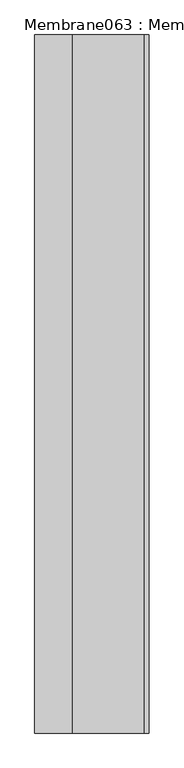
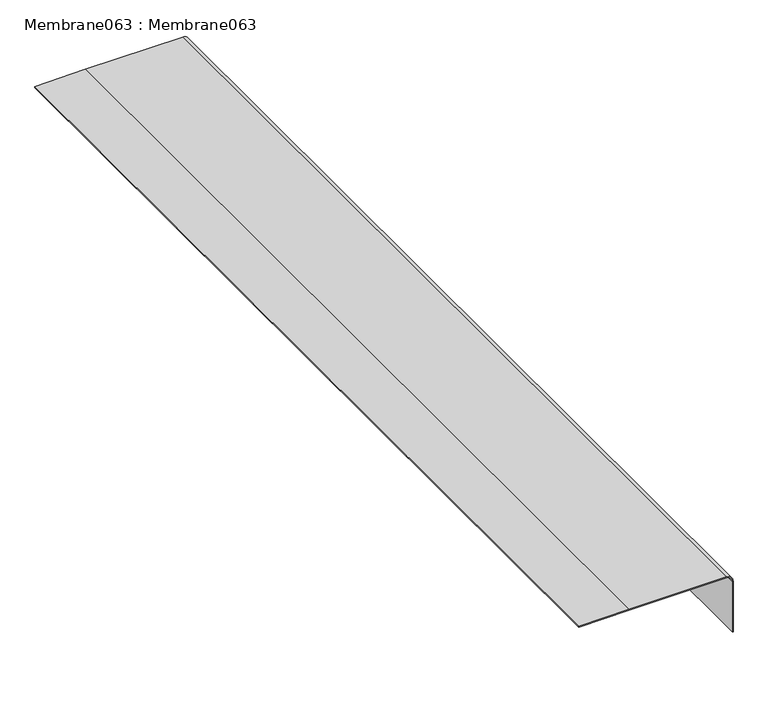
"""IFC4 building model written with IfcOpenShell, lengths in millimetres: proxy geometry, Membrane063 : Membrane063."""

from ifc_helpers import new_model, si_unit, point, frame, frame_2d, origin, place, context, project, spatial, polyline, circle_curve, trimmed, segment, composite_curve, outline, extrude, source, transform, mapped, element, save


def membrane063_membrane063_a49dec39(model_context):
    return source(origin(), model_context, "Body", "SweptSolid", [
        extrude(outline(composite_curve([segment(polyline([(40234.5370749, -4374.0545197), (40120.9129128, -4374.0545197), (40120.9129128, -4372.0545197), (40234.5370749, -4372.0545197)]), True, "CONTINUOUS"), segment(trimmed(circle_curve(frame_2d((40234.5370749, -4386.0545197)), 14.0), [point((40234.5370749, -4372.0545197))], [point((40248.5370749, -4386.0545197))], False, "CARTESIAN"), True, "CONTINUOUS"), segment(polyline([(40248.5370749, -4386.0545197), (40248.5370749, -4593.337414), (40247.0048323, -4699.8063764), (40245.0046252, -4699.8063764), (40246.5370749, -4593.3230233), (40246.5370749, -4386.0545197)]), True, "CONTINUOUS"), segment(trimmed(circle_curve(frame_2d((40234.5370749, -4386.0545197)), 12.0), [point((40246.5370749, -4386.0545197))], [point((40234.5370749, -4374.0545197))], True, "CARTESIAN"), True, "CONTINUOUS")], self_intersect=False)), frame((0.0, -1052.8906574, 0.0), z_axis=(0.0, 1.0, 0.0), x_axis=(0.0, 0.0, 1.0)), (0.0, 0.0, 1.0), 2000.0),
    ])


if __name__ == "__main__":
    model = new_model("IFC4")
    model_context = context("Model", 3, world=origin())
    ifc_project = project(units=[si_unit("LENGTHUNIT", "METRE", prefix="MILLI")], contexts=[model_context])
    site = spatial("IfcSite", under=ifc_project)
    building = spatial("IfcBuilding", under=site)
    placement = place(None, origin())
    membrane063_membrane063_shape = membrane063_membrane063_a49dec39(model_context)
    element("IfcBuildingElementProxy", 1, Name="Membrane063 : Membrane063", ObjectType="Membrane063 : Membrane063", at=placement, inside=building, context=model_context, shape_type="MappedRepresentation", body=[
        mapped(membrane063_membrane063_shape, transform((0.0, 0.0, 0.0), x_axis=(1.0, 0.0, 0.0), y_axis=(0.0, 1.0, 0.0), z_axis=(0.0, 0.0, 1.0))),
    ])
    save(model, "model.ifc")

# Revit data of these elements
# Type "Membrane063 : Membrane063"
#   NameOverride = "Membrane063"
# Element 1 (IfcBuildingElementProxy, "Membrane063 : Membrane063")
#   Materials on its faces: "THREE PLY BUILT UP ROOF MEMBRANE"
# Materials
#   "THREE PLY BUILT UP ROOF MEMBRANE": class "Unassigned", colour RGB 63 63 63, transparency 0
